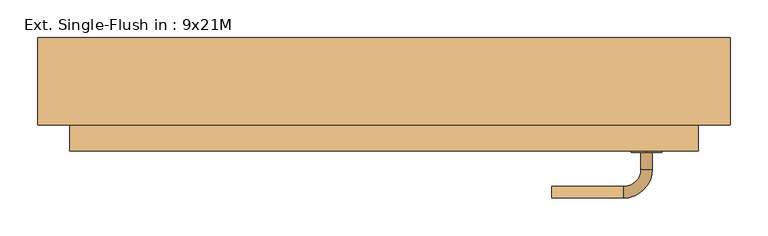
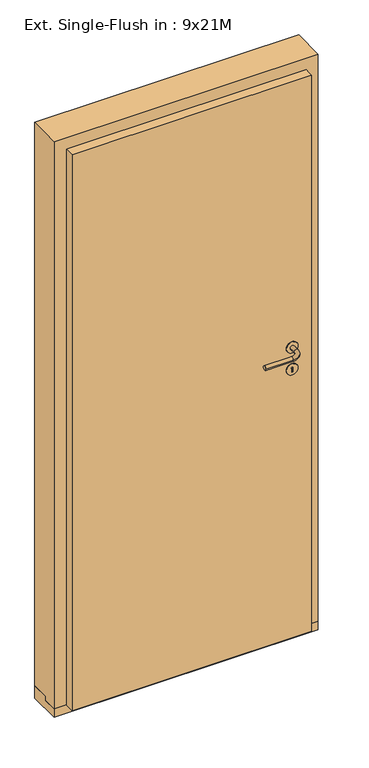
"""IFC4 building model written with IfcOpenShell, lengths in millimetres: door geometry, Ext. Single-Flush in : 9x21M."""

from ifc_helpers import new_model, si_unit, point, frame, frame_2d, origin, place, context, project, spatial, polyline, circle_curve, ellipse_curve, trimmed, segment, composite_curve, outline, extrude, faceted_brep, source, transform, mapped, element, save
from ifc_brep_helpers import plane_surface, cylinder_surface, revolved_surface, advanced_brep


def ext_single_flush_in_9x21m_d6ab10a1(model_context):
    return source(origin(), model_context, "Body", "SolidModel", [
        extrude(outline(composite_curve([segment(trimmed(circle_curve(frame_2d((1090.0, 346.0)), 20.0), [point((1070.0, 346.0))], [point((1110.0, 346.0))], False, "CARTESIAN"), True, "CONTINUOUS"), segment(trimmed(circle_curve(frame_2d((1090.0, 346.0)), 20.0), [point((1110.0, 346.0))], [point((1070.0, 346.0))], False, "CARTESIAN"), True, "CONTINUOUS")], self_intersect=False)), frame((0.0, 33.0, 0.0), z_axis=(0.0, 1.0, 0.0), x_axis=(0.0, 0.0, 1.0)), (0.0, 0.0, 1.0), 2.0),
        advanced_brep(
        [(353.5, 33.0, 1090.0), (338.5, 33.0, 1090.0), (353.5, 10.5, 1090.0), (338.5, 10.5, 1090.0), (316.0, -12.0, 1090.0), (316.0, -27.0, 1090.0), (221.0, -27.0, 1090.0), (221.0, -12.0, 1090.0)],
        [
            (0, 1, circle_curve(frame((346.0, 33.0, 1090.0), z_axis=(0.0, 1.0, 0.0), x_axis=(-1.0, 0.0, 0.0)), 7.5)),
            (1, 0, circle_curve(frame((346.0, 33.0, 1090.0), z_axis=(0.0, 1.0, 0.0), x_axis=(-1.0, 0.0, 0.0)), 7.5)),
            (0, 2),
            (2, 3, circle_curve(frame((346.0, 10.5, 1090.0), z_axis=(0.0, 1.0, 0.0), x_axis=(-1.0, 0.0, 0.0)), 7.5)),
            (3, 1),
            (3, 2, circle_curve(frame((346.0, 10.5, 1090.0), z_axis=(0.0, 1.0, 0.0), x_axis=(-1.0, 0.0, 0.0)), 7.5)),
            (4, 3, circle_curve(frame((316.0, 10.5, 1090.0), z_axis=(0.0, 0.0, 1.0), x_axis=(1.0, 0.0, 0.0)), 22.5)),
            (2, 5, circle_curve(frame((316.0, 10.5, 1090.0), z_axis=(0.0, 0.0, -1.0), x_axis=(1.0, 0.0, 0.0)), 37.5)),
            (5, 4, circle_curve(frame((316.0, -19.5, 1090.0), z_axis=(1.0, 0.0, 0.0), x_axis=(0.0, 1.0, 0.0)), 7.5)),
            (4, 5, circle_curve(frame((316.0, -19.5, 1090.0), z_axis=(1.0, 0.0, 0.0), x_axis=(0.0, 1.0, 0.0)), 7.5)),
            (5, 6),
            (6, 7, circle_curve(frame((221.0, -19.5, 1090.0), z_axis=(1.0, 0.0, 0.0), x_axis=(0.0, 1.0, 0.0)), 7.5)),
            (7, 4),
            (7, 6, circle_curve(frame((221.0, -19.5, 1090.0), z_axis=(1.0, 0.0, 0.0), x_axis=(0.0, 1.0, 0.0)), 7.5)),
        ],
        [
            plane_surface(frame((346.0, 33.0, 1090.0), z_axis=(0.0, 1.0, 0.0), x_axis=(0.0, 0.0, -1.0))),
            cylinder_surface(frame((346.0, 33.0, 1090.0), z_axis=(0.0, 1.0, 0.0), x_axis=(-1.0, 0.0, 0.0)), 7.5),
            revolved_surface(trimmed(ellipse_curve(frame((346.0, 10.5, 1090.0), z_axis=(0.0, 1.0, 0.0), x_axis=(-1.0, 0.0, 0.0)), 7.5, 7.5), [point((353.5, 10.5, 1090.0))], [point((338.5, 10.5, 1090.0))], True, "CARTESIAN"), (316.0, 10.5, 1090.0), (0.0, 0.0, -1.0)),
            revolved_surface(trimmed(ellipse_curve(frame((346.0, 10.5, 1090.0), z_axis=(0.0, 1.0, 0.0), x_axis=(-1.0, 0.0, 0.0)), 7.5, 7.5), [point((338.5, 10.5, 1090.0))], [point((353.5, 10.5, 1090.0))], True, "CARTESIAN"), (316.0, 10.5, 1090.0), (0.0, 0.0, -1.0)),
            cylinder_surface(frame((316.0, -19.5, 1090.0), z_axis=(1.0, 0.0, 0.0), x_axis=(0.0, 1.0, 0.0)), 7.5),
            plane_surface(frame((221.0, -19.5, 1090.0), z_axis=(-1.0, 0.0, 0.0), x_axis=(0.0, 0.0, -1.0))),
        ],
        [
            (0, [[1, 2]]),
            (1, [[-1, 3, 4, 5]]),
            (1, [[-2, -5, 6, -3]]),
            (2, [[7, -4, 8, 9]]),
            (3, [[-8, -6, -7, 10]]),
            (4, [[-9, 11, 12, 13]]),
            (4, [[-10, -13, 14, -11]]),
            (5, [[-14, -12]]),
        ],
    ),
        extrude(outline(composite_curve([segment(trimmed(circle_curve(frame_2d((1010.0, 346.0)), 20.0), [point((990.0, 346.0))], [point((1030.0, 346.0))], False, "CARTESIAN"), True, "CONTINUOUS"), segment(trimmed(circle_curve(frame_2d((1010.0, 346.0)), 20.0), [point((1030.0, 346.0))], [point((990.0, 346.0))], False, "CARTESIAN"), True, "CONTINUOUS")], self_intersect=False), holes=[composite_curve([segment(polyline([(1012.4019238, 347.5), (1000.0, 347.5), (1000.0, 344.5), (1012.4019238, 344.5)]), True, "CONTINUOUS"), segment(trimmed(circle_curve(frame_2d((1015.0, 346.0)), 3.0), [point((1012.4019238, 344.5))], [point((1012.4019238, 347.5))], True, "CARTESIAN"), True, "CONTINUOUS")], self_intersect=False)]), frame((0.0, 33.0, 0.0), z_axis=(0.0, 1.0, 0.0), x_axis=(0.0, 0.0, 1.0)), (0.0, 0.0, 1.0), 2.0),
        extrude(outline(composite_curve([segment(trimmed(circle_curve(frame_2d((1090.0, 346.0)), 20.0), [point((1070.0, 346.0))], [point((1110.0, 346.0))], False, "CARTESIAN"), True, "CONTINUOUS"), segment(trimmed(circle_curve(frame_2d((1090.0, 346.0)), 20.0), [point((1110.0, 346.0))], [point((1070.0, 346.0))], False, "CARTESIAN"), True, "CONTINUOUS")], self_intersect=False)), frame((0.0, 85.0, 0.0), z_axis=(0.0, 1.0, 0.0), x_axis=(0.0, 0.0, 1.0)), (0.0, 0.0, 1.0), 2.0),
        advanced_brep(
        [(353.5, 87.0, 1090.0), (338.5, 87.0, 1090.0), (338.5, 109.5, 1090.0), (353.5, 109.5, 1090.0), (316.0, 132.0, 1090.0), (316.0, 147.0, 1090.0), (221.0, 132.0, 1090.0), (221.0, 147.0, 1090.0)],
        [
            (0, 1, circle_curve(frame((346.0, 87.0, 1090.0), z_axis=(0.0, -1.0, 0.0), x_axis=(-1.0, 0.0, 0.0)), 7.5)),
            (1, 0, circle_curve(frame((346.0, 87.0, 1090.0), z_axis=(0.0, -1.0, 0.0), x_axis=(-1.0, 0.0, 0.0)), 7.5)),
            (1, 2),
            (2, 3, circle_curve(frame((346.0, 109.5, 1090.0), z_axis=(0.0, -1.0, 0.0), x_axis=(-1.0, 0.0, 0.0)), 7.5)),
            (3, 0),
            (3, 2, circle_curve(frame((346.0, 109.5, 1090.0), z_axis=(0.0, -1.0, 0.0), x_axis=(-1.0, 0.0, 0.0)), 7.5)),
            (4, 5, circle_curve(frame((316.0, 139.5, 1090.0), z_axis=(1.0, 0.0, 0.0), x_axis=(0.0, -1.0, 0.0)), 7.5)),
            (5, 3, circle_curve(frame((316.0, 109.5, 1090.0), z_axis=(0.0, 0.0, -1.0), x_axis=(1.0, 0.0, 0.0)), 37.5)),
            (2, 4, circle_curve(frame((316.0, 109.5, 1090.0), z_axis=(0.0, 0.0, 1.0), x_axis=(1.0, 0.0, 0.0)), 22.5)),
            (5, 4, circle_curve(frame((316.0, 139.5, 1090.0), z_axis=(1.0, 0.0, 0.0), x_axis=(0.0, -1.0, 0.0)), 7.5)),
            (4, 6),
            (6, 7, circle_curve(frame((221.0, 139.5, 1090.0), z_axis=(1.0, 0.0, 0.0), x_axis=(0.0, -1.0, 0.0)), 7.5)),
            (7, 5),
            (7, 6, circle_curve(frame((221.0, 139.5, 1090.0), z_axis=(1.0, 0.0, 0.0), x_axis=(0.0, -1.0, 0.0)), 7.5)),
        ],
        [
            plane_surface(frame((346.0, 87.0, 1090.0), z_axis=(0.0, -1.0, 0.0), x_axis=(0.0, 0.0, -1.0))),
            cylinder_surface(frame((346.0, 87.0, 1090.0), z_axis=(0.0, -1.0, 0.0), x_axis=(-1.0, 0.0, 0.0)), 7.5),
            revolved_surface(trimmed(ellipse_curve(frame((346.0, 109.5, 1090.0), z_axis=(0.0, 1.0, 0.0), x_axis=(-1.0, 0.0, 0.0)), 7.5, 7.5), [point((353.5, 109.5, 1090.0))], [point((338.5, 109.5, 1090.0))], True, "CARTESIAN"), (316.0, 109.5, 1090.0), (0.0, 0.0, -1.0)),
            revolved_surface(trimmed(ellipse_curve(frame((346.0, 109.5, 1090.0), z_axis=(0.0, 1.0, 0.0), x_axis=(-1.0, 0.0, 0.0)), 7.5, 7.5), [point((338.5, 109.5, 1090.0))], [point((353.5, 109.5, 1090.0))], True, "CARTESIAN"), (316.0, 109.5, 1090.0), (0.0, 0.0, -1.0)),
            cylinder_surface(frame((316.0, 139.5, 1090.0), z_axis=(1.0, 0.0, 0.0), x_axis=(0.0, -1.0, 0.0)), 7.5),
            plane_surface(frame((221.0, 139.5, 1090.0), z_axis=(-1.0, 0.0, 0.0), x_axis=(0.0, 0.0, -1.0))),
        ],
        [
            (0, [[1, 2]]),
            (1, [[3, 4, 5, -2]]),
            (1, [[-5, 6, -3, -1]]),
            (2, [[7, 8, -4, 9]]),
            (3, [[10, -9, -6, -8]]),
            (4, [[11, 12, 13, -7]]),
            (4, [[-13, 14, -11, -10]]),
            (5, [[-12, -14]]),
        ],
    ),
        extrude(outline(composite_curve([segment(trimmed(circle_curve(frame_2d((1010.0, 346.0)), 20.0), [point((990.0, 346.0))], [point((1030.0, 346.0))], False, "CARTESIAN"), True, "CONTINUOUS"), segment(trimmed(circle_curve(frame_2d((1010.0, 346.0)), 20.0), [point((1030.0, 346.0))], [point((990.0, 346.0))], False, "CARTESIAN"), True, "CONTINUOUS")], self_intersect=False), holes=[composite_curve([segment(polyline([(1012.4019238, 347.5), (1000.0, 347.5), (1000.0, 344.5), (1012.4019238, 344.5)]), True, "CONTINUOUS"), segment(trimmed(circle_curve(frame_2d((1015.0, 346.0)), 3.0), [point((1012.4019238, 344.5))], [point((1012.4019238, 347.5))], True, "CARTESIAN"), True, "CONTINUOUS")], self_intersect=False)]), frame((0.0, 85.0, 0.0), z_axis=(0.0, 1.0, 0.0), x_axis=(0.0, 0.0, 1.0)), (0.0, 0.0, 1.0), 2.0),
        faceted_brep([(-414.0, 69.0, 2058.0), (414.0, 69.0, 2058.0), (414.0, 69.0, 30.0), (456.0, 69.0, 30.0), (456.0, 69.0, 2100.0), (-456.0, 69.0, 2100.0), (-456.0, 69.0, 30.0), (-414.0, 69.0, 30.0), (414.0, 119.0, 2058.0), (414.0, 119.0, 45.0), (414.0, 119.0, 30.0), (-456.0, 119.0, 30.0), (-414.0, 119.0, 30.0), (456.0, 119.0, 30.0), (456.0, 184.0, 2100.0), (456.0, 119.0, 45.0), (456.0, 184.0, 45.0), (-456.0, 184.0, 2100.0), (-456.0, 184.0, 45.0), (-456.0, 119.0, 45.0), (-414.0, 119.0, 2058.0), (-414.0, 119.0, 45.0), (399.0, 184.0, 45.0), (399.0, 184.0, 2043.0), (-399.0, 184.0, 2043.0), (-399.0, 184.0, 45.0), (-399.0, 119.0, 45.0), (399.0, 119.0, 45.0), (399.0, 119.0, 2043.0), (-399.0, 119.0, 2043.0)], [[[0, 1, 2, 3, 4, 5, 6, 7]], [[1, 8, 9, 10, 2]], [[11, 12, 7, 6]], [[10, 13, 3, 2]], [[14, 4, 3, 13, 15, 16]], [[5, 17, 18, 19, 11, 6]], [[20, 0, 7, 12, 21]], [[17, 14, 16, 22, 23, 24, 25, 18]], [[21, 19, 18, 25, 26]], [[15, 9, 27, 22, 16]], [[12, 11, 19, 21]], [[13, 10, 9, 15]], [[28, 23, 22, 27]], [[24, 29, 26, 25]], [[29, 28, 27, 9, 8, 20, 21, 26]], [[5, 4, 14, 17]], [[24, 23, 28, 29]], [[1, 0, 20, 8]]]),
        extrude(outline(polyline([(-414.0, 85.0), (414.0, 85.0), (414.0, 35.0), (-414.0, 35.0), (-414.0, 85.0)])), frame((0.0, 0.0, 30.0), z_axis=(0.0, 0.0, 1.0), x_axis=(1.0, 0.0, 0.0)), (0.0, 0.0, 1.0), 2028.0),
        extrude(outline(polyline([(69.0, 30.0), (119.0, 30.0), (119.0, 45.0), (184.0, 45.0), (184.0, 0.0), (69.0, 0.0), (69.0, 30.0)])), frame((-456.0, 0.0, 0.0), z_axis=(1.0, 0.0, 0.0), x_axis=(0.0, 1.0, 0.0)), (0.0, 0.0, 1.0), 912.0),
    ])


if __name__ == "__main__":
    model = new_model("IFC4")
    model_context = context("Model", 3, world=origin())
    ifc_project = project(units=[si_unit("LENGTHUNIT", "METRE", prefix="MILLI")], contexts=[model_context])
    site = spatial("IfcSite", under=ifc_project)
    building = spatial("IfcBuilding", under=site)
    placement = place(None, origin())
    ext_single_flush_in_9x21m_shape = ext_single_flush_in_9x21m_d6ab10a1(model_context)
    element("IfcDoor", 1, ObjectType="Ext. Single-Flush in : 9x21M", at=placement, inside=building, context=model_context, shape_type="MappedRepresentation", body=[
        mapped(ext_single_flush_in_9x21m_shape, transform((0.0, 0.0, 0.0), x_axis=(1.0, 0.0, 0.0), y_axis=(0.0, 1.0, 0.0), z_axis=(0.0, 0.0, 1.0))),
    ])
    save(model, "model.ifc")

# Revit data of these elements
# Type "Ext. Single-Flush in : 9x21M"
#   Type Mark = "62"
#   Sound Rating = ""
#   Opening Side [instance default] = "in"
#   Hinge Side [instance default] = ""
#   Creator Build [instance default] = "2017.0301.0"
#   Creator Organization [instance default] = "© Danish Educational Content"
#   Creator Name [instance default] = "© Erik Falck Jørgensen"
#   Analytic Construction = "<None>"
#   length#5 = 912 mm
#   length#4 = 120 mm
#   length#3 = 30 mm
#   length#2 = 57 mm
#   length#1 = 0 mm
#   Thickness = 50 mm
#   Seal Width = 12 mm
#   Rough Width = 912 mm
#   Rough Height = 2100 mm
#   Rebate Depth = 50 mm
#   Rabbet Width = 15 mm
#   Rabbet Depth = 50 mm
#   Height = 2088 mm
#   Width = 888 mm
#   Handle From Side = 110 mm
#   Handle From Bottom = 1090 mm
#   Exterior Direction [instance default] = 0.00°
#   Case Depth = 115 mm
#   Case Width = 45 mm
#   Threshold = yes
#   Sealing = no
#   Hinging = yes
#   Wall Closure = 1
#   Function = 1
#   Panel = none
#   Handle Finish = none
#   Handle = element 628255
#   Case/Transom = none
#   Assembly Code = ""
# Element 1 (IfcDoor, "Ext. Single-Flush in : 9x21M")
#   Materials on its faces: "Stainless Steel, Polished", "Default Frame/Mullion (Interior/Exterior)", "Default Door Panel (Exterior/Interior)"
# Materials
#   "Stainless Steel, Polished": class "Metal", colour RGB 180 180 180, transparency 0, Description = "Rustfri stål, poleret", Cost = 0
#   "Default Frame/Mullion (Interior/Exterior)": class "Generic", colour RGB 205 205 205, transparency 0, Description = "Udefineret karm/ramme materiale", Cost = 0
#   "Default Door Panel (Exterior/Interior)": class "Generic", colour RGB 205 205 205, transparency 0, Description = "Udefineret dørplade materiale", Cost = 0
